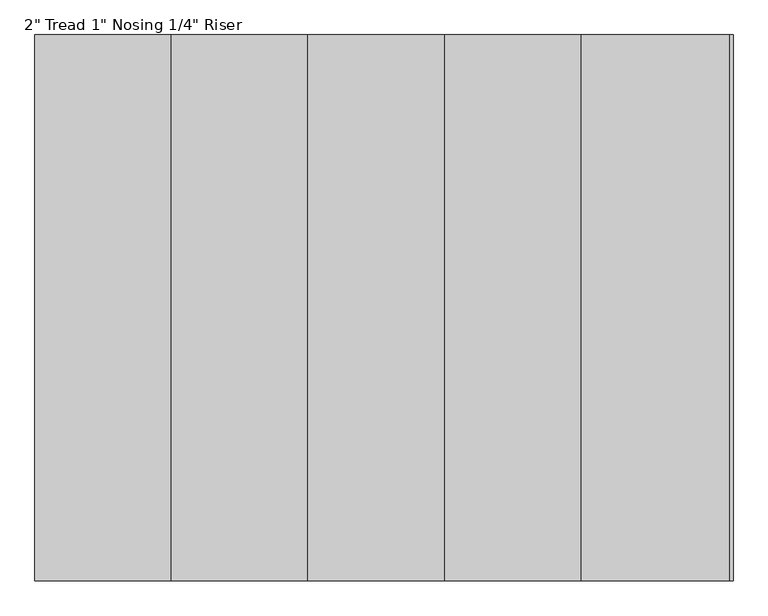
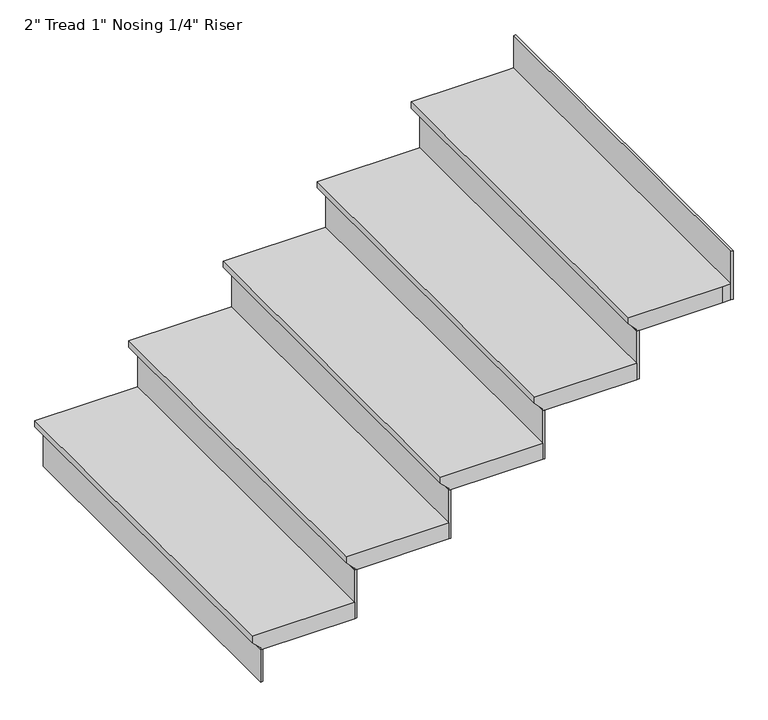
"""IFC4 building model written with IfcOpenShell, lengths in millimetres: stair flight geometry."""

from ifc_helpers import new_model, si_unit, origin, place, context, project, spatial, faceted_brep, source, transform, mapped, element, save


def stair_flight_71736acc(model_context):
    return source(origin(), model_context, "Body", "Brep", [
        faceted_brep([(-2715.2122732, 8132.6265304, -781.05), (-2715.2122732, 8132.6265304, -762.0), (-2715.2122732, 9250.2265304, -762.0), (-2715.2122732, 9250.2265304, -781.05), (-2689.8122732, 8132.6265304, -806.45), (-2689.8122732, 9250.2265304, -806.45), (-2410.4122732, 8132.6265304, -762.0), (-2410.4122732, 9250.2265304, -762.0), (-2689.8122732, 9250.2265304, -812.8), (-2410.4122732, 9250.2265304, -812.8), (-2410.4122732, 8132.6265304, -812.8), (-2689.8122732, 8132.6265304, -812.8)], [[[0, 1, 2, 3]], [[4, 0, 3, 5]], [[2, 1, 6, 7]], [[8, 9, 10, 11]], [[2, 7, 9, 8, 5, 3]], [[8, 11, 4, 5]], [[6, 1, 0, 4, 11, 10]], [[7, 6, 10, 9]]]),
        faceted_brep([(-2689.8122732, 8132.6265304, -812.8), (-2689.8122732, 8132.6265304, -914.4), (-2683.4622732, 8132.6265304, -914.4), (-2683.4622732, 8132.6265304, -812.8), (-2689.8122732, 9250.2265304, -812.8), (-2683.4622732, 9250.2265304, -812.8), (-2683.4622732, 9250.2265304, -914.4), (-2689.8122732, 9250.2265304, -914.4)], [[[0, 1, 2, 3]], [[4, 5, 6, 7]], [[1, 0, 4, 7]], [[2, 1, 7, 6]], [[3, 2, 6, 5]], [[0, 3, 5, 4]]]),
        faceted_brep([(-2410.4122732, 8132.6265304, -660.4), (-2410.4122732, 8132.6265304, -812.8), (-2404.0622732, 8132.6265304, -812.8), (-2404.0622732, 8132.6265304, -660.4), (-2410.4122732, 9250.2265304, -660.4), (-2404.0622732, 9250.2265304, -660.4), (-2404.0622732, 9250.2265304, -812.8), (-2410.4122732, 9250.2265304, -812.8)], [[[0, 1, 2, 3]], [[4, 5, 6, 7]], [[1, 0, 4, 7]], [[2, 1, 7, 6]], [[3, 2, 6, 5]], [[0, 3, 5, 4]]]),
        faceted_brep([(-2435.8122732, 9250.2265304, -609.6), (-2435.8122732, 8132.6265304, -609.6), (-2131.0122732, 8132.6265304, -609.6), (-2131.0122732, 9250.2265304, -609.6), (-2410.4122732, 9250.2265304, -660.4), (-2131.0122732, 9250.2265304, -660.4), (-2131.0122732, 8132.6265304, -660.4), (-2410.4122732, 8132.6265304, -660.4), (-2410.4122732, 9250.2265304, -654.05), (-2435.8122732, 9250.2265304, -628.65), (-2410.4122732, 8132.6265304, -654.05), (-2435.8122732, 8132.6265304, -628.65)], [[[0, 1, 2, 3]], [[4, 5, 6, 7]], [[0, 3, 5, 4, 8, 9]], [[4, 7, 10, 8]], [[2, 1, 11, 10, 7, 6]], [[3, 2, 6, 5]], [[11, 1, 0, 9]], [[10, 11, 9, 8]]]),
        faceted_brep([(-2131.0122732, 8132.6265304, -508.0), (-2131.0122732, 8132.6265304, -660.4), (-2124.6622732, 8132.6265304, -660.4), (-2124.6622732, 8132.6265304, -508.0), (-2131.0122732, 9250.2265304, -508.0), (-2124.6622732, 9250.2265304, -508.0), (-2124.6622732, 9250.2265304, -660.4), (-2131.0122732, 9250.2265304, -660.4)], [[[0, 1, 2, 3]], [[4, 5, 6, 7]], [[1, 0, 4, 7]], [[2, 1, 7, 6]], [[3, 2, 6, 5]], [[0, 3, 5, 4]]]),
        faceted_brep([(-2156.4122732, 9250.2265304, -457.2), (-2156.4122732, 8132.6265304, -457.2), (-1851.6122732, 8132.6265304, -457.2), (-1851.6122732, 9250.2265304, -457.2), (-2131.0122732, 9250.2265304, -508.0), (-1851.6122732, 9250.2265304, -508.0), (-1851.6122732, 8132.6265304, -508.0), (-2131.0122732, 8132.6265304, -508.0), (-2131.0122732, 9250.2265304, -501.65), (-2156.4122732, 9250.2265304, -476.25), (-2131.0122732, 8132.6265304, -501.65), (-2156.4122732, 8132.6265304, -476.25)], [[[0, 1, 2, 3]], [[4, 5, 6, 7]], [[0, 3, 5, 4, 8, 9]], [[4, 7, 10, 8]], [[2, 1, 11, 10, 7, 6]], [[3, 2, 6, 5]], [[11, 1, 0, 9]], [[10, 11, 9, 8]]]),
        faceted_brep([(-1851.6122732, 8132.6265304, -355.6), (-1851.6122732, 8132.6265304, -508.0), (-1845.2622732, 8132.6265304, -508.0), (-1845.2622732, 8132.6265304, -355.6), (-1851.6122732, 9250.2265304, -355.6), (-1845.2622732, 9250.2265304, -355.6), (-1845.2622732, 9250.2265304, -508.0), (-1851.6122732, 9250.2265304, -508.0)], [[[0, 1, 2, 3]], [[4, 5, 6, 7]], [[1, 0, 4, 7]], [[2, 1, 7, 6]], [[3, 2, 6, 5]], [[0, 3, 5, 4]]]),
        faceted_brep([(-1877.0122732, 9250.2265304, -304.8), (-1877.0122732, 8132.6265304, -304.8), (-1572.2122732, 8132.6265304, -304.8), (-1572.2122732, 9250.2265304, -304.8), (-1851.6122732, 9250.2265304, -355.6), (-1572.2122732, 9250.2265304, -355.6), (-1572.2122732, 8132.6265304, -355.6), (-1851.6122732, 8132.6265304, -355.6), (-1851.6122732, 9250.2265304, -349.25), (-1877.0122732, 9250.2265304, -323.85), (-1851.6122732, 8132.6265304, -349.25), (-1877.0122732, 8132.6265304, -323.85)], [[[0, 1, 2, 3]], [[4, 5, 6, 7]], [[0, 3, 5, 4, 8, 9]], [[4, 7, 10, 8]], [[2, 1, 11, 10, 7, 6]], [[3, 2, 6, 5]], [[11, 1, 0, 9]], [[10, 11, 9, 8]]]),
        faceted_brep([(-1292.8122732, 8132.6265304, -50.8), (-1292.8122732, 8132.6265304, -203.2), (-1286.4622732, 8132.6265304, -203.2), (-1286.4622732, 8132.6265304, -50.8), (-1292.8122732, 9250.2265304, -50.8), (-1286.4622732, 9250.2265304, -50.8), (-1286.4622732, 9250.2265304, -203.2), (-1292.8122732, 9250.2265304, -203.2)], [[[0, 1, 2, 3]], [[4, 5, 6, 7]], [[1, 0, 4, 7]], [[2, 1, 7, 6]], [[3, 2, 6, 5]], [[0, 3, 5, 4]]]),
        faceted_brep([(-1572.2122732, 8132.6265304, -203.2), (-1572.2122732, 8132.6265304, -355.6), (-1565.8622732, 8132.6265304, -355.6), (-1565.8622732, 8132.6265304, -203.2), (-1572.2122732, 9250.2265304, -203.2), (-1565.8622732, 9250.2265304, -203.2), (-1565.8622732, 9250.2265304, -355.6), (-1572.2122732, 9250.2265304, -355.6)], [[[0, 1, 2, 3]], [[4, 5, 6, 7]], [[1, 0, 4, 7]], [[2, 1, 7, 6]], [[3, 2, 6, 5]], [[0, 3, 5, 4]]]),
        faceted_brep([(-1292.8122732, 9250.2265304, -152.4), (-1318.2122732, 9250.2265304, -152.4), (-1597.6122732, 9250.2265304, -152.4), (-1597.6122732, 8132.6265304, -152.4), (-1318.2122732, 8132.6265304, -152.4), (-1292.8122732, 8132.6265304, -152.4), (-1318.2122732, 9250.2265304, -203.2), (-1292.8122732, 9250.2265304, -203.2), (-1292.8122732, 8132.6265304, -203.2), (-1318.2122732, 8132.6265304, -203.2), (-1572.2122732, 8132.6265304, -203.2), (-1572.2122732, 9250.2265304, -203.2), (-1572.2122732, 9250.2265304, -196.85), (-1597.6122732, 9250.2265304, -171.45), (-1572.2122732, 8132.6265304, -196.85), (-1597.6122732, 8132.6265304, -171.45)], [[[0, 1, 2, 3, 4, 5]], [[6, 7, 8, 9, 10, 11]], [[1, 0, 7, 6]], [[2, 1, 6, 11, 12, 13]], [[11, 10, 14, 12]], [[4, 3, 15, 14, 10, 9]], [[5, 4, 9, 8]], [[0, 5, 8, 7]], [[15, 3, 2, 13]], [[14, 15, 13, 12]]]),
    ])


if __name__ == "__main__":
    model = new_model("IFC4")
    model_context = context("Model", 3, world=origin())
    ifc_project = project(units=[si_unit("LENGTHUNIT", "METRE", prefix="MILLI")], contexts=[model_context])
    site = spatial("IfcSite", under=ifc_project)
    building = spatial("IfcBuilding", under=site)
    placement = place(None, origin())
    stair_flight_shape = stair_flight_71736acc(model_context)
    element("IfcStairFlight", 1, ObjectType="2\" Tread 1\" Nosing 1/4\" Riser", at=placement, inside=building, context=model_context, shape_type="MappedRepresentation", body=[
        mapped(stair_flight_shape, transform((0.0, 0.0, 0.0), x_axis=(1.0, 0.0, 0.0), y_axis=(0.0, 1.0, 0.0), z_axis=(0.0, 0.0, 1.0))),
    ])
    save(model, "model.ifc")
